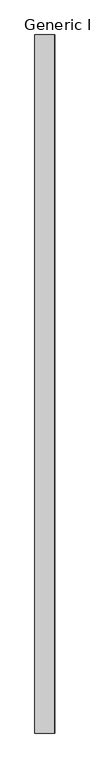
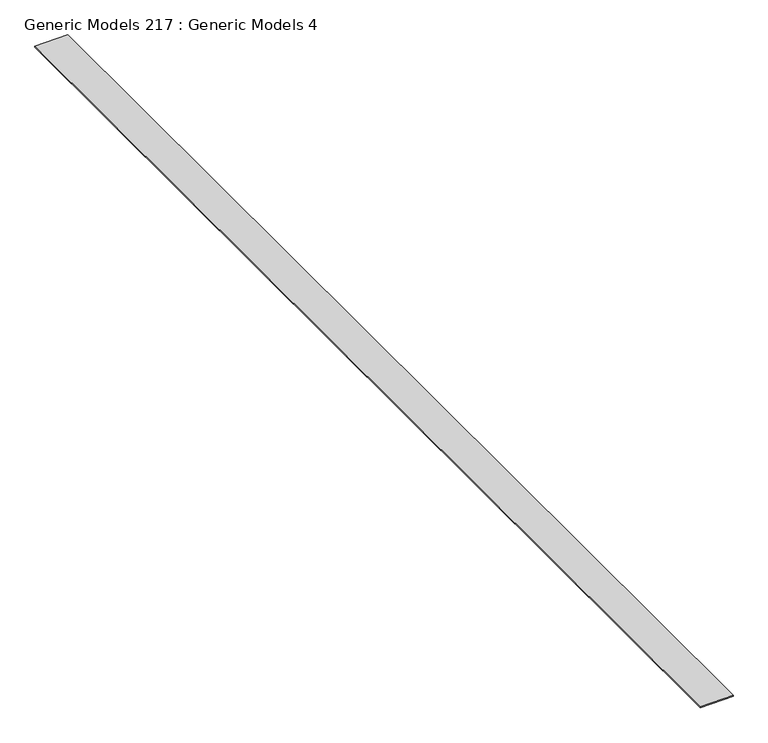
"""IFC4 building model written with IfcOpenShell, lengths in millimetres: proxy geometry, Generic Models 217 : Generic Models 4."""

from ifc_helpers import new_model, si_unit, frame, origin, place, context, project, spatial, polyline, outline, extrude, source, transform, mapped, element, save


def generic_models_217_generic_models_4_47b4c880(model_context):
    return source(origin(), model_context, "Body", "SweptSolid", [
        extrude(outline(polyline([(0.0, -532.7341933), (0.0, 0.0), (18643.6, 0.0), (18643.6, -532.7341933), (0.0, -532.7341933)])), frame((7853.8190325, -6864.9230338, 126907.7313143), z_axis=(-0.020828813681888794, 0.0, 0.9997830567281111), x_axis=(0.0, 1.0, 0.0)), (0.0, 0.0, 1.0), 12.7),
    ])


if __name__ == "__main__":
    model = new_model("IFC4")
    model_context = context("Model", 3, world=origin())
    ifc_project = project(units=[si_unit("LENGTHUNIT", "METRE", prefix="MILLI")], contexts=[model_context])
    site = spatial("IfcSite", under=ifc_project)
    building = spatial("IfcBuilding", under=site)
    placement = place(None, origin())
    generic_models_217_generic_models_4_shape = generic_models_217_generic_models_4_47b4c880(model_context)
    element("IfcBuildingElementProxy", 1, Name="Generic Models 217 : Generic Models 4", ObjectType="Generic Models 217 : Generic Models 4", at=placement, inside=building, context=model_context, shape_type="MappedRepresentation", body=[
        mapped(generic_models_217_generic_models_4_shape, transform((0.0, 0.0, 0.0), x_axis=(1.0, 0.0, 0.0), y_axis=(0.0, 1.0, 0.0), z_axis=(0.0, 0.0, 1.0))),
    ])
    save(model, "model.ifc")

# Revit data of these elements
# Element 1 (IfcBuildingElementProxy, "Generic Models 217 : Generic Models 4")
#   Materials on its faces: "_1/2\" CDX PLYWOOD"
# Materials
#   "_1/2\" CDX PLYWOOD": class "Generic", colour RGB 98 75 74, transparency 0, Cost = 0
